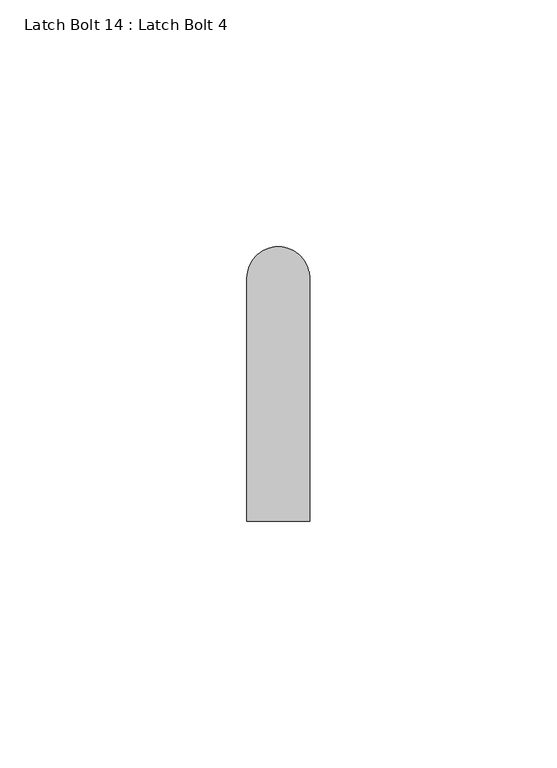
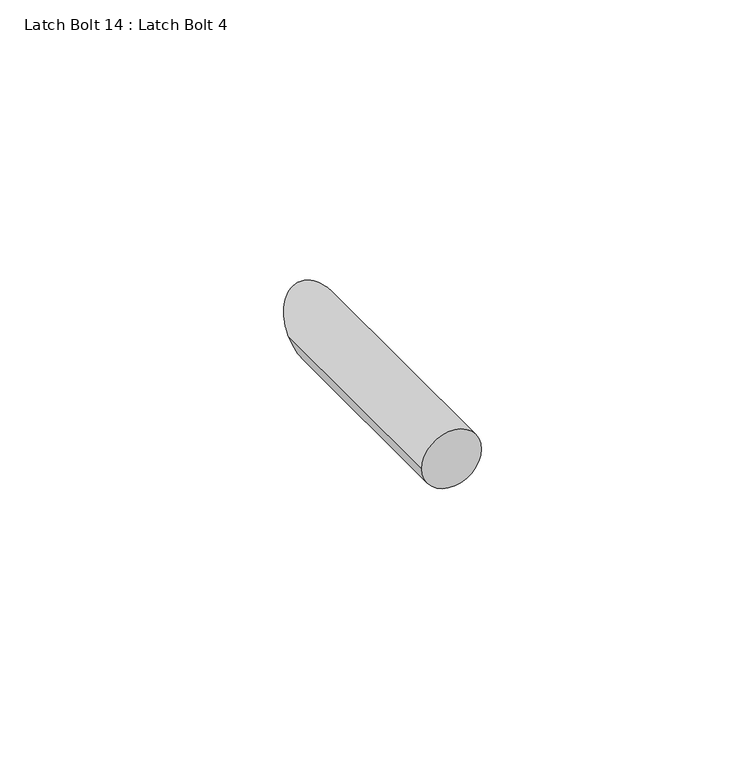
"""IFC4 building model written with IfcOpenShell, lengths in millimetres: proxy geometry, Latch Bolt 14 : Latch Bolt 4."""

import ifcopenshell
import ifcopenshell.guid

model = None  # the IFC model being written
_history = None  # IfcOwnerHistory: only IFC2X3 demands one
_inside = {}  # id of a spatial element -> (the spatial element, [elements in it])
_under = {}  # id of a project, library or spatial element -> (it, [spatial elements below it])
_declared = {}  # id of a project -> (the project, [libraries it declares])
_typed = {}  # id of a type object -> (the type object, [elements of that type])
_made_of = {}  # id of a material, layer set ... -> (it, [elements and type objects made of it])


def new_model(schema):
    """Start an empty IFC model of exactly this schema.

    Asked for "IFC4X3", IfcOpenShell would pick the latest addendum, in which some entities
    have other attributes; the version numbers below select the first issue.
    IFC2X3 requires an IfcOwnerHistory on every rooted entity: one is made here for all.
    """
    global model, _history
    if schema == "IFC4X3":
        model = ifcopenshell.file(schema_version=(4, 3, 0, 0))
    else:
        model = ifcopenshell.file(schema=schema)
    _inside.clear()
    _under.clear()
    _declared.clear()
    _typed.clear()
    _made_of.clear()
    _history = None
    if model.schema == "IFC2X3":
        org = make("IfcOrganization", Name="unknown")
        user = make(
            "IfcPersonAndOrganization",
            ThePerson=make("IfcPerson", FamilyName="unknown"),
            TheOrganization=org,
        )
        app = make(
            "IfcApplication",
            ApplicationDeveloper=org,
            Version="unknown",
            ApplicationFullName="unknown",
            ApplicationIdentifier="unknown",
        )
        _history = make(
            "IfcOwnerHistory",
            OwningUser=user,
            OwningApplication=app,
            ChangeAction="ADDED",
            CreationDate=0,
        )
    return model


def make(cls, **values):
    """One entity of the class cls with the attributes given. An attribute that is None is left unset."""
    return model.create_entity(
        cls, **{name: value for name, value in values.items() if value is not None}
    )


def rooted(cls, **values):
    """An entity with a GlobalId (a new one), such as an element, a storey or a relation."""
    return make(cls, GlobalId=ifcopenshell.guid.new(), OwnerHistory=_history, **values)


def si_unit(unit_type, name, prefix=None):
    """IfcSIUnit, for example si_unit("LENGTHUNIT", "METRE", prefix="MILLI")."""
    return make("IfcSIUnit", UnitType=unit_type, Prefix=prefix, Name=name)


def assignment(units):
    """IfcUnitAssignment: the units of a project."""
    return None if units is None else make("IfcUnitAssignment", Units=units)


def point(xyz):
    """IfcCartesianPoint."""
    return None if xyz is None else make("IfcCartesianPoint", Coordinates=xyz)


def direction(xyz):
    """IfcDirection."""
    return None if xyz is None else make("IfcDirection", DirectionRatios=xyz)


def frame(location, z_axis=None, x_axis=None):
    """IfcAxis2Placement3D, a coordinate frame: its origin and axes. An axis left out is left unset."""
    return make(
        "IfcAxis2Placement3D",
        Location=point(location),
        Axis=direction(z_axis),
        RefDirection=direction(x_axis),
    )


def origin():
    """The frame at (0, 0, 0) with its axes left unset."""
    return frame((0.0, 0.0, 0.0))


def place(relative_to, where):
    """IfcLocalPlacement: puts the frame where relative to a parent placement (None: the world)."""
    return make(
        "IfcLocalPlacement", PlacementRelTo=relative_to, RelativePlacement=where
    )


def context(
    kind, dimensions, precision=None, world=None, true_north=None, identifier=None
):
    """IfcGeometricRepresentationContext, for example the 3D "Model" context."""
    return make(
        "IfcGeometricRepresentationContext",
        ContextIdentifier=identifier,
        ContextType=kind,
        CoordinateSpaceDimension=dimensions,
        Precision=precision,
        WorldCoordinateSystem=world,
        TrueNorth=true_north,
    )


def project(units=None, contexts=None):
    """IfcProject with its units and contexts."""
    return rooted(
        "IfcProject",
        Name="project",
        RepresentationContexts=contexts,
        UnitsInContext=assignment(units),
    )


def spatial(cls, under=None, at=None, **own):
    """A site, building, storey or space (cls), placed at a placement, below another one or the project."""
    s = rooted(cls, ObjectPlacement=at, **own)
    if under is not None:
        _under.setdefault(under.id(), (under, []))[1].append(s)
    return s


def circle_curve(where, radius):
    """IfcCircle in the frame where."""
    return make("IfcCircle", Position=where, Radius=radius)


def ellipse_curve(where, semi_axis1, semi_axis2):
    """IfcEllipse in the frame where."""
    return make(
        "IfcEllipse", Position=where, SemiAxis1=semi_axis1, SemiAxis2=semi_axis2
    )


def shape(context_of_items, identifier, shape_type, items):
    """IfcShapeRepresentation: the items that make up one representation, for example the "Body"."""
    return make(
        "IfcShapeRepresentation",
        ContextOfItems=context_of_items,
        RepresentationIdentifier=identifier,
        RepresentationType=shape_type,
        Items=items,
    )


def source(mapping_origin, context_of_items, identifier, shape_type, items):
    """IfcRepresentationMap: a shape defined once, which mapped items show again and again."""
    return make(
        "IfcRepresentationMap",
        MappingOrigin=mapping_origin,
        MappedRepresentation=shape(context_of_items, identifier, shape_type, items),
    )


def transform(
    local_origin,
    x_axis=None,
    y_axis=None,
    z_axis=None,
    scale=None,
    scale2=None,
    scale3=None,
    uniform=True,
):
    """IfcCartesianTransformationOperator3D, or its non-uniform kind. x_axis, y_axis, z_axis: its Axis1, 2, 3."""
    if uniform:
        return make(
            "IfcCartesianTransformationOperator3D",
            Axis1=direction(x_axis),
            Axis2=direction(y_axis),
            LocalOrigin=point(local_origin),
            Scale=scale,
            Axis3=direction(z_axis),
        )
    return make(
        "IfcCartesianTransformationOperator3DnonUniform",
        Axis1=direction(x_axis),
        Axis2=direction(y_axis),
        LocalOrigin=point(local_origin),
        Scale=scale,
        Axis3=direction(z_axis),
        Scale2=scale2,
        Scale3=scale3,
    )


def mapped(mapping_source, mapping_target):
    """IfcMappedItem: shows the shape of a source again, moved by a transform."""
    return make(
        "IfcMappedItem", MappingSource=mapping_source, MappingTarget=mapping_target
    )


def made_of(thing, what):
    """Note that an element or type object is made of a material, layer set ...; save() writes the relation."""
    if what is not None:
        _made_of.setdefault(what.id(), (what, []))[1].append(thing)
    return thing


def element(
    cls,
    number,
    at=None,
    inside=None,
    cuts=None,
    type_object=None,
    material=None,
    context=None,
    identifier="Body",
    shape_type=None,
    held_by="IfcProductDefinitionShape",
    body=None,
    shapes=None,
    **own,
):
    """One element of the class cls, such as IfcWall. Its Tag is "e" and its number.

    at: its placement. inside: the storey or other place that contains it. cuts: it is an
    opening in that element (IfcRelVoidsElement). A single representation is given by context,
    identifier, shape_type and body (its items); several are given by shapes. held_by: the class
    of the entity that holds the representations. save() writes the other relations.
    """
    e = rooted(cls, Tag="e%d" % number, ObjectPlacement=at, **own)
    if body is not None:
        shapes = [shape(context, identifier, shape_type, body)]
    if shapes is not None:
        e.Representation = make(held_by, Representations=shapes)
    if inside is not None:
        _inside.setdefault(inside.id(), (inside, []))[1].append(e)
    if cuts is not None:
        rooted(
            "IfcRelVoidsElement", RelatingBuildingElement=cuts, RelatedOpeningElement=e
        )
    if type_object is not None:
        _typed.setdefault(type_object.id(), (type_object, []))[1].append(e)
    return made_of(e, material)


def aggregate(whole, parts):
    """IfcRelAggregates: a whole, such as a stair, and the parts it consists of."""
    return rooted("IfcRelAggregates", RelatingObject=whole, RelatedObjects=parts)


def save(model, path):
    """Write the relations noted so far, then the file.

    IfcRelAggregates (storeys below a building ...), IfcRelContainedInSpatialStructure (elements
    in a storey), IfcRelDefinesByType, IfcRelAssociatesMaterial and IfcRelDeclares: one each for
    every whole, place, type object, material and project.
    """
    for whole, parts in _under.values():
        aggregate(whole, parts)
    for where, things in _inside.values():
        rooted(
            "IfcRelContainedInSpatialStructure",
            RelatedElements=things,
            RelatingStructure=where,
        )
    for kind, things in _typed.values():
        rooted("IfcRelDefinesByType", RelatedObjects=things, RelatingType=kind)
    for what, things in _made_of.values():
        rooted("IfcRelAssociatesMaterial", RelatedObjects=things, RelatingMaterial=what)
    for by, libraries in _declared.values():
        rooted("IfcRelDeclares", RelatingContext=by, RelatedDefinitions=libraries)
    model.write(path)


def plane_surface(at):
    """IfcPlane: the flat surface through the origin of the frame at, square to its z axis."""
    return make("IfcPlane", Position=at)


def cylinder_surface(at, radius):
    """IfcCylindricalSurface: all points at the distance radius from the z axis of the frame at."""
    return make("IfcCylindricalSurface", Position=at, Radius=radius)


def advanced_brep(points, edges, surfaces, faces):
    """IfcAdvancedBrep: a solid bounded by faces that lie on surfaces and meet in shared edges.

    An edge is (start, end): straight between two places in points (the first is 0);
    or (start, end, curve); or (start, end, curve, False) where it runs against its curve.
    A face is (place in surfaces, loops), or (place, loops, False) where it looks against
    its surface's normal. A loop lists edges by number (the first is 1), with a minus sign
    where the edge is run from its end to its start. The first loop is the outer one.
    """
    corners = [point(p) for p in points]
    vertices = [make("IfcVertexPoint", VertexGeometry=c) for c in corners]
    made = []
    for start, end, *more in edges:
        made.append(
            make(
                "IfcEdgeCurve",
                EdgeStart=vertices[start],
                EdgeEnd=vertices[end],
                EdgeGeometry=more[0] if more else make("IfcPolyline", Points=[corners[start], corners[end]]),
                SameSense=more[1] if len(more) > 1 else True,
            )
        )
    hull = []
    for where, loops, *sense in faces:
        bounds = []
        for j, loop in enumerate(loops):
            ring = [make("IfcOrientedEdge", EdgeElement=made[abs(k) - 1], Orientation=k > 0) for k in loop]
            bounds.append(
                make(
                    "IfcFaceOuterBound" if j == 0 else "IfcFaceBound",
                    Bound=make("IfcEdgeLoop", EdgeList=ring),
                    Orientation=True,
                )
            )
        hull.append(make("IfcAdvancedFace", Bounds=bounds, FaceSurface=surfaces[where], SameSense=sense[0] if sense else True))
    return make("IfcAdvancedBrep", Outer=make("IfcClosedShell", CfsFaces=hull))


def latch_bolt_14_latch_bolt_4_7b3a1efd(model_context):
    return source(origin(), model_context, "Body", "AdvancedBrep", [
        advanced_brep(
        [(587315.8935739, -535212.6610985, 292.1), (587303.1935739, -535212.6610985, 292.1), (587315.8935739, -535163.4485985, 292.1), (587303.1935739, -535163.4485985, 292.1)],
        [
            (0, 1, circle_curve(frame((587309.5435739, -535212.6610985, 292.1), z_axis=(0.0, -1.0, 0.0), x_axis=(1.0, 0.0, 0.0)), 6.35)),
            (1, 0, circle_curve(frame((587309.5435739, -535212.6610985, 292.1), z_axis=(0.0, -1.0, 0.0), x_axis=(1.0, 0.0, 0.0)), 6.35)),
            (0, 2),
            (2, 3, ellipse_curve(frame((587309.5435739, -535163.4485985, 292.1), z_axis=(0.0, -0.7071067811865497, 0.7071067811865455), x_axis=(0.0, -0.7071067811865454, -0.7071067811865497)), 8.9802561, 6.35)),
            (3, 1),
            (3, 2, ellipse_curve(frame((587309.5435739, -535163.4485985, 292.1), z_axis=(0.0, -0.7071067811865497, 0.7071067811865455), x_axis=(0.0, -0.7071067811865454, -0.7071067811865497)), 8.9802561, 6.35)),
        ],
        [
            plane_surface(frame((587315.8935739, -535212.6610985, 292.1), z_axis=(0.0, -1.0, 0.0), x_axis=(0.0, 0.0, 1.0))),
            cylinder_surface(frame((587309.5435739, -535155.5110985, 292.1), z_axis=(0.0, -1.0, 0.0), x_axis=(1.0, 0.0, 0.0)), 6.35),
            plane_surface(frame((587338.1185739, -535171.3860985, 284.1625), z_axis=(0.0, 0.7071067811865497, -0.7071067811865455), x_axis=(-1.0, 0.0, 0.0))),
        ],
        [
            (0, [[1, 2]]),
            (1, [[-1, 3, 4, 5]]),
            (1, [[-2, -5, 6, -3]]),
            (2, [[-4, -6]]),
        ],
    ),
    ])


if __name__ == "__main__":
    model = new_model("IFC4")
    model_context = context("Model", 3, world=origin())
    ifc_project = project(units=[si_unit("LENGTHUNIT", "METRE", prefix="MILLI")], contexts=[model_context])
    site = spatial("IfcSite", under=ifc_project)
    building = spatial("IfcBuilding", under=site)
    placement = place(None, origin())
    latch_bolt_14_latch_bolt_4_shape = latch_bolt_14_latch_bolt_4_7b3a1efd(model_context)
    element("IfcBuildingElementProxy", 1, Name="Latch Bolt 14 : Latch Bolt 4", ObjectType="Latch Bolt 14 : Latch Bolt 4", at=placement, inside=building, context=model_context, shape_type="MappedRepresentation", body=[
        mapped(latch_bolt_14_latch_bolt_4_shape, transform((0.0, 0.0, 0.0), x_axis=(1.0, 0.0, 0.0), y_axis=(0.0, 1.0, 0.0), z_axis=(0.0, 0.0, 1.0))),
    ])
    save(model, "model.ifc")

# Revit data of these elements
# Element 1 (IfcBuildingElementProxy, "Latch Bolt 14 : Latch Bolt 4")
#   Materials on its faces: "GALV. SLIDE BOLT"
# Materials
#   "GALV. SLIDE BOLT": class "Metal", colour RGB 189 187 185, transparency 0, Description = "Carbon steel", Cost = 0
